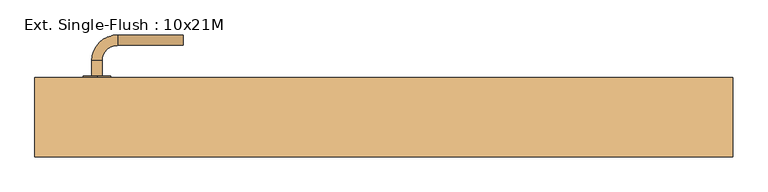
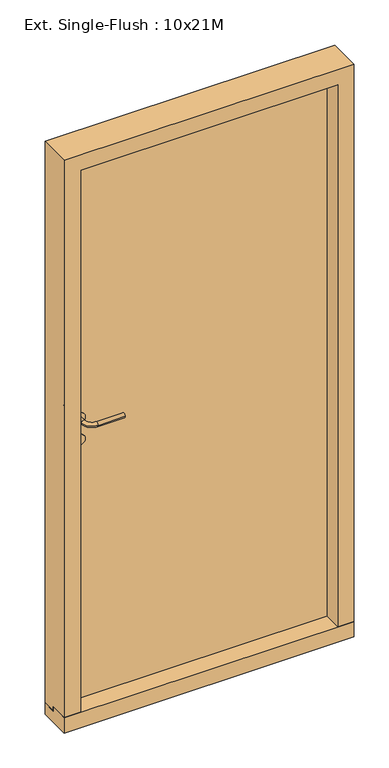
"""IFC4 building model written with IfcOpenShell, lengths in millimetres: door geometry, Ext. Single-Flush : 10x21M."""

import ifcopenshell
import ifcopenshell.guid

model = None  # the IFC model being written
_history = None  # IfcOwnerHistory: only IFC2X3 demands one
_inside = {}  # id of a spatial element -> (the spatial element, [elements in it])
_under = {}  # id of a project, library or spatial element -> (it, [spatial elements below it])
_declared = {}  # id of a project -> (the project, [libraries it declares])
_typed = {}  # id of a type object -> (the type object, [elements of that type])
_made_of = {}  # id of a material, layer set ... -> (it, [elements and type objects made of it])


def new_model(schema):
    """Start an empty IFC model of exactly this schema.

    Asked for "IFC4X3", IfcOpenShell would pick the latest addendum, in which some entities
    have other attributes; the version numbers below select the first issue.
    IFC2X3 requires an IfcOwnerHistory on every rooted entity: one is made here for all.
    """
    global model, _history
    if schema == "IFC4X3":
        model = ifcopenshell.file(schema_version=(4, 3, 0, 0))
    else:
        model = ifcopenshell.file(schema=schema)
    _inside.clear()
    _under.clear()
    _declared.clear()
    _typed.clear()
    _made_of.clear()
    _history = None
    if model.schema == "IFC2X3":
        org = make("IfcOrganization", Name="unknown")
        user = make(
            "IfcPersonAndOrganization",
            ThePerson=make("IfcPerson", FamilyName="unknown"),
            TheOrganization=org,
        )
        app = make(
            "IfcApplication",
            ApplicationDeveloper=org,
            Version="unknown",
            ApplicationFullName="unknown",
            ApplicationIdentifier="unknown",
        )
        _history = make(
            "IfcOwnerHistory",
            OwningUser=user,
            OwningApplication=app,
            ChangeAction="ADDED",
            CreationDate=0,
        )
    return model


def make(cls, **values):
    """One entity of the class cls with the attributes given. An attribute that is None is left unset."""
    return model.create_entity(
        cls, **{name: value for name, value in values.items() if value is not None}
    )


def rooted(cls, **values):
    """An entity with a GlobalId (a new one), such as an element, a storey or a relation."""
    return make(cls, GlobalId=ifcopenshell.guid.new(), OwnerHistory=_history, **values)


def si_unit(unit_type, name, prefix=None):
    """IfcSIUnit, for example si_unit("LENGTHUNIT", "METRE", prefix="MILLI")."""
    return make("IfcSIUnit", UnitType=unit_type, Prefix=prefix, Name=name)


def assignment(units):
    """IfcUnitAssignment: the units of a project."""
    return None if units is None else make("IfcUnitAssignment", Units=units)


def point(xyz):
    """IfcCartesianPoint."""
    return None if xyz is None else make("IfcCartesianPoint", Coordinates=xyz)


def direction(xyz):
    """IfcDirection."""
    return None if xyz is None else make("IfcDirection", DirectionRatios=xyz)


def frame(location, z_axis=None, x_axis=None):
    """IfcAxis2Placement3D, a coordinate frame: its origin and axes. An axis left out is left unset."""
    return make(
        "IfcAxis2Placement3D",
        Location=point(location),
        Axis=direction(z_axis),
        RefDirection=direction(x_axis),
    )


def frame_2d(location, x_axis=None):
    """IfcAxis2Placement2D, a coordinate frame in the plane: its origin and x axis."""
    return make(
        "IfcAxis2Placement2D", Location=point(location), RefDirection=direction(x_axis)
    )


def origin():
    """The frame at (0, 0, 0) with its axes left unset."""
    return frame((0.0, 0.0, 0.0))


def place(relative_to, where):
    """IfcLocalPlacement: puts the frame where relative to a parent placement (None: the world)."""
    return make(
        "IfcLocalPlacement", PlacementRelTo=relative_to, RelativePlacement=where
    )


def context(
    kind, dimensions, precision=None, world=None, true_north=None, identifier=None
):
    """IfcGeometricRepresentationContext, for example the 3D "Model" context."""
    return make(
        "IfcGeometricRepresentationContext",
        ContextIdentifier=identifier,
        ContextType=kind,
        CoordinateSpaceDimension=dimensions,
        Precision=precision,
        WorldCoordinateSystem=world,
        TrueNorth=true_north,
    )


def project(units=None, contexts=None):
    """IfcProject with its units and contexts."""
    return rooted(
        "IfcProject",
        Name="project",
        RepresentationContexts=contexts,
        UnitsInContext=assignment(units),
    )


def spatial(cls, under=None, at=None, **own):
    """A site, building, storey or space (cls), placed at a placement, below another one or the project."""
    s = rooted(cls, ObjectPlacement=at, **own)
    if under is not None:
        _under.setdefault(under.id(), (under, []))[1].append(s)
    return s


def polyline(points):
    """IfcPolyline through the points."""
    return make("IfcPolyline", Points=[point(p) for p in points])


def circle_curve(where, radius):
    """IfcCircle in the frame where."""
    return make("IfcCircle", Position=where, Radius=radius)


def ellipse_curve(where, semi_axis1, semi_axis2):
    """IfcEllipse in the frame where."""
    return make(
        "IfcEllipse", Position=where, SemiAxis1=semi_axis1, SemiAxis2=semi_axis2
    )


def trimmed(basis, trim1, trim2, sense, master):
    """IfcTrimmedCurve: the piece of a basis curve between two trims."""
    return make(
        "IfcTrimmedCurve",
        BasisCurve=basis,
        Trim1=trim1,
        Trim2=trim2,
        SenseAgreement=sense,
        MasterRepresentation=master,
    )


def segment(curve, same_sense, transition):
    """IfcCompositeCurveSegment."""
    return make(
        "IfcCompositeCurveSegment",
        Transition=transition,
        SameSense=same_sense,
        ParentCurve=curve,
    )


def composite_curve(segments, self_intersect=None):
    """IfcCompositeCurve: segments joined end to end."""
    return make("IfcCompositeCurve", Segments=segments, SelfIntersect=self_intersect)


def outline(outer, holes=None, kind="AREA"):
    """IfcArbitraryClosedProfileDef: a profile drawn as a closed curve; with holes, ...WithVoids."""
    if holes is None:
        return make("IfcArbitraryClosedProfileDef", ProfileType=kind, OuterCurve=outer)
    return make(
        "IfcArbitraryProfileDefWithVoids",
        ProfileType=kind,
        OuterCurve=outer,
        InnerCurves=holes,
    )


def extrude(swept, where, along, depth):
    """IfcExtrudedAreaSolid: the profile swept, set in the frame where, extruded along a direction by depth."""
    return make(
        "IfcExtrudedAreaSolid",
        SweptArea=swept,
        Position=where,
        ExtrudedDirection=direction(along),
        Depth=depth,
    )


def faces_of(points, faces, orient=None, outer=None):
    """IfcFace entities. A face is a list of loops; a loop is a list of indices into points, from 0.

    orient and outer hold one flag for each loop. By default every Orientation is true, the
    first loop of a face is its IfcFaceOuterBound and the others are IfcFaceBound.
    """
    made = []
    for i, loops in enumerate(faces):
        bounds = []
        for j, loop in enumerate(loops):
            is_outer = j == 0 if outer is None else outer[i][j]
            bounds.append(
                make(
                    "IfcFaceOuterBound" if is_outer else "IfcFaceBound",
                    Bound=make("IfcPolyLoop", Polygon=[points[k] for k in loop]),
                    Orientation=True if orient is None else orient[i][j],
                )
            )
        made.append(make("IfcFace", Bounds=bounds))
    return made


def faceted_brep(points, faces, orient=None, outer=None, voids=None):
    """IfcFacetedBrep: a solid bounded by flat faces; with voids (closed shells), ...WithVoids."""
    shared = [point(p) for p in points]
    hull = make("IfcClosedShell", CfsFaces=faces_of(shared, faces, orient, outer))
    if voids is None:
        return make("IfcFacetedBrep", Outer=hull)
    return make(
        "IfcFacetedBrepWithVoids",
        Outer=hull,
        Voids=[
            make(cls, CfsFaces=faces_of(shared, fs, o, b)) for cls, fs, o, b in voids
        ],
    )


def shape(context_of_items, identifier, shape_type, items):
    """IfcShapeRepresentation: the items that make up one representation, for example the "Body"."""
    return make(
        "IfcShapeRepresentation",
        ContextOfItems=context_of_items,
        RepresentationIdentifier=identifier,
        RepresentationType=shape_type,
        Items=items,
    )


def source(mapping_origin, context_of_items, identifier, shape_type, items):
    """IfcRepresentationMap: a shape defined once, which mapped items show again and again."""
    return make(
        "IfcRepresentationMap",
        MappingOrigin=mapping_origin,
        MappedRepresentation=shape(context_of_items, identifier, shape_type, items),
    )


def transform(
    local_origin,
    x_axis=None,
    y_axis=None,
    z_axis=None,
    scale=None,
    scale2=None,
    scale3=None,
    uniform=True,
):
    """IfcCartesianTransformationOperator3D, or its non-uniform kind. x_axis, y_axis, z_axis: its Axis1, 2, 3."""
    if uniform:
        return make(
            "IfcCartesianTransformationOperator3D",
            Axis1=direction(x_axis),
            Axis2=direction(y_axis),
            LocalOrigin=point(local_origin),
            Scale=scale,
            Axis3=direction(z_axis),
        )
    return make(
        "IfcCartesianTransformationOperator3DnonUniform",
        Axis1=direction(x_axis),
        Axis2=direction(y_axis),
        LocalOrigin=point(local_origin),
        Scale=scale,
        Axis3=direction(z_axis),
        Scale2=scale2,
        Scale3=scale3,
    )


def mapped(mapping_source, mapping_target):
    """IfcMappedItem: shows the shape of a source again, moved by a transform."""
    return make(
        "IfcMappedItem", MappingSource=mapping_source, MappingTarget=mapping_target
    )


def made_of(thing, what):
    """Note that an element or type object is made of a material, layer set ...; save() writes the relation."""
    if what is not None:
        _made_of.setdefault(what.id(), (what, []))[1].append(thing)
    return thing


def element(
    cls,
    number,
    at=None,
    inside=None,
    cuts=None,
    type_object=None,
    material=None,
    context=None,
    identifier="Body",
    shape_type=None,
    held_by="IfcProductDefinitionShape",
    body=None,
    shapes=None,
    **own,
):
    """One element of the class cls, such as IfcWall. Its Tag is "e" and its number.

    at: its placement. inside: the storey or other place that contains it. cuts: it is an
    opening in that element (IfcRelVoidsElement). A single representation is given by context,
    identifier, shape_type and body (its items); several are given by shapes. held_by: the class
    of the entity that holds the representations. save() writes the other relations.
    """
    e = rooted(cls, Tag="e%d" % number, ObjectPlacement=at, **own)
    if body is not None:
        shapes = [shape(context, identifier, shape_type, body)]
    if shapes is not None:
        e.Representation = make(held_by, Representations=shapes)
    if inside is not None:
        _inside.setdefault(inside.id(), (inside, []))[1].append(e)
    if cuts is not None:
        rooted(
            "IfcRelVoidsElement", RelatingBuildingElement=cuts, RelatedOpeningElement=e
        )
    if type_object is not None:
        _typed.setdefault(type_object.id(), (type_object, []))[1].append(e)
    return made_of(e, material)


def aggregate(whole, parts):
    """IfcRelAggregates: a whole, such as a stair, and the parts it consists of."""
    return rooted("IfcRelAggregates", RelatingObject=whole, RelatedObjects=parts)


def save(model, path):
    """Write the relations noted so far, then the file.

    IfcRelAggregates (storeys below a building ...), IfcRelContainedInSpatialStructure (elements
    in a storey), IfcRelDefinesByType, IfcRelAssociatesMaterial and IfcRelDeclares: one each for
    every whole, place, type object, material and project.
    """
    for whole, parts in _under.values():
        aggregate(whole, parts)
    for where, things in _inside.values():
        rooted(
            "IfcRelContainedInSpatialStructure",
            RelatedElements=things,
            RelatingStructure=where,
        )
    for kind, things in _typed.values():
        rooted("IfcRelDefinesByType", RelatedObjects=things, RelatingType=kind)
    for what, things in _made_of.values():
        rooted("IfcRelAssociatesMaterial", RelatedObjects=things, RelatingMaterial=what)
    for by, libraries in _declared.values():
        rooted("IfcRelDeclares", RelatingContext=by, RelatedDefinitions=libraries)
    model.write(path)


def plane_surface(at):
    """IfcPlane: the flat surface through the origin of the frame at, square to its z axis."""
    return make("IfcPlane", Position=at)


def cylinder_surface(at, radius):
    """IfcCylindricalSurface: all points at the distance radius from the z axis of the frame at."""
    return make("IfcCylindricalSurface", Position=at, Radius=radius)


def revolved_surface(curve, axis_point, axis_direction):
    """IfcSurfaceOfRevolution: the curve turned about the line through axis_point along axis_direction."""
    return make(
        "IfcSurfaceOfRevolution",
        SweptCurve=make("IfcArbitraryOpenProfileDef", ProfileType="CURVE", Curve=curve),
        AxisPosition=make("IfcAxis1Placement", Location=point(axis_point), Axis=direction(axis_direction)),
    )


def advanced_brep(points, edges, surfaces, faces):
    """IfcAdvancedBrep: a solid bounded by faces that lie on surfaces and meet in shared edges.

    An edge is (start, end): straight between two places in points (the first is 0);
    or (start, end, curve); or (start, end, curve, False) where it runs against its curve.
    A face is (place in surfaces, loops), or (place, loops, False) where it looks against
    its surface's normal. A loop lists edges by number (the first is 1), with a minus sign
    where the edge is run from its end to its start. The first loop is the outer one.
    """
    corners = [point(p) for p in points]
    vertices = [make("IfcVertexPoint", VertexGeometry=c) for c in corners]
    made = []
    for start, end, *more in edges:
        made.append(
            make(
                "IfcEdgeCurve",
                EdgeStart=vertices[start],
                EdgeEnd=vertices[end],
                EdgeGeometry=more[0] if more else make("IfcPolyline", Points=[corners[start], corners[end]]),
                SameSense=more[1] if len(more) > 1 else True,
            )
        )
    hull = []
    for where, loops, *sense in faces:
        bounds = []
        for j, loop in enumerate(loops):
            ring = [make("IfcOrientedEdge", EdgeElement=made[abs(k) - 1], Orientation=k > 0) for k in loop]
            bounds.append(
                make(
                    "IfcFaceOuterBound" if j == 0 else "IfcFaceBound",
                    Bound=make("IfcEdgeLoop", EdgeList=ring),
                    Orientation=True,
                )
            )
        hull.append(make("IfcAdvancedFace", Bounds=bounds, FaceSurface=surfaces[where], SameSense=sense[0] if sense else True))
    return make("IfcAdvancedBrep", Outer=make("IfcClosedShell", CfsFaces=hull))


def ext_single_flush_10x21m_d0052ec9(model_context):
    return source(origin(), model_context, "Body", "SolidModel", [
        extrude(outline(composite_curve([segment(trimmed(circle_curve(frame_2d((1090.0, -416.0)), 20.0), [point((1070.0, -416.0))], [point((1110.0, -416.0))], False, "CARTESIAN"), True, "CONTINUOUS"), segment(trimmed(circle_curve(frame_2d((1090.0, -416.0)), 20.0), [point((1110.0, -416.0))], [point((1070.0, -416.0))], False, "CARTESIAN"), True, "CONTINUOUS")], self_intersect=False)), frame((0.0, 184.0, 0.0), z_axis=(0.0, 1.0, 0.0), x_axis=(0.0, 0.0, 1.0)), (0.0, 0.0, 1.0), 2.0),
        advanced_brep(
        [(-423.5, 186.0, 1090.0), (-408.5, 186.0, 1090.0), (-423.5, 208.5, 1090.0), (-408.5, 208.5, 1090.0), (-386.0, 231.0, 1090.0), (-386.0, 246.0, 1090.0), (-291.0, 246.0, 1090.0), (-291.0, 231.0, 1090.0)],
        [
            (0, 1, circle_curve(frame((-416.0, 186.0, 1090.0), z_axis=(0.0, -1.0, 0.0), x_axis=(1.0, 0.0, 0.0)), 7.5)),
            (1, 0, circle_curve(frame((-416.0, 186.0, 1090.0), z_axis=(0.0, -1.0, 0.0), x_axis=(1.0, 0.0, 0.0)), 7.5)),
            (0, 2),
            (2, 3, circle_curve(frame((-416.0, 208.5, 1090.0), z_axis=(0.0, -1.0, 0.0), x_axis=(1.0, 0.0, 0.0)), 7.5)),
            (3, 1),
            (3, 2, circle_curve(frame((-416.0, 208.5, 1090.0), z_axis=(0.0, -1.0, 0.0), x_axis=(1.0, 0.0, 0.0)), 7.5)),
            (4, 3, circle_curve(frame((-386.0, 208.5, 1090.0), z_axis=(0.0, 0.0, 1.0), x_axis=(-1.0, 0.0, 0.0)), 22.5)),
            (2, 5, circle_curve(frame((-386.0, 208.5, 1090.0), z_axis=(0.0, 0.0, -1.0), x_axis=(-1.0, 0.0, 0.0)), 37.5)),
            (5, 4, circle_curve(frame((-386.0, 238.5, 1090.0), z_axis=(-1.0, 0.0, 0.0), x_axis=(0.0, -1.0, 0.0)), 7.5)),
            (4, 5, circle_curve(frame((-386.0, 238.5, 1090.0), z_axis=(-1.0, 0.0, 0.0), x_axis=(0.0, -1.0, 0.0)), 7.5)),
            (5, 6),
            (6, 7, circle_curve(frame((-291.0, 238.5, 1090.0), z_axis=(-1.0, 0.0, 0.0), x_axis=(0.0, -1.0, 0.0)), 7.5)),
            (7, 4),
            (7, 6, circle_curve(frame((-291.0, 238.5, 1090.0), z_axis=(-1.0, 0.0, 0.0), x_axis=(0.0, -1.0, 0.0)), 7.5)),
        ],
        [
            plane_surface(frame((-416.0, 186.0, 1090.0), z_axis=(0.0, -1.0, 0.0), x_axis=(0.0, 0.0, -1.0))),
            cylinder_surface(frame((-416.0, 186.0, 1090.0), z_axis=(0.0, -1.0, 0.0), x_axis=(1.0, 0.0, 0.0)), 7.5),
            revolved_surface(trimmed(ellipse_curve(frame((-416.0, 208.5, 1090.0), z_axis=(0.0, -1.0, 0.0), x_axis=(1.0, 0.0, 0.0)), 7.5, 7.5), [point((-423.5, 208.5, 1090.0))], [point((-408.5, 208.5, 1090.0))], True, "CARTESIAN"), (-386.0, 208.5, 1090.0), (0.0, 0.0, -1.0)),
            revolved_surface(trimmed(ellipse_curve(frame((-416.0, 208.5, 1090.0), z_axis=(0.0, -1.0, 0.0), x_axis=(1.0, 0.0, 0.0)), 7.5, 7.5), [point((-408.5, 208.5, 1090.0))], [point((-423.5, 208.5, 1090.0))], True, "CARTESIAN"), (-386.0, 208.5, 1090.0), (0.0, 0.0, -1.0)),
            cylinder_surface(frame((-386.0, 238.5, 1090.0), z_axis=(-1.0, 0.0, 0.0), x_axis=(0.0, -1.0, 0.0)), 7.5),
            plane_surface(frame((-291.0, 238.5, 1090.0), z_axis=(1.0, 0.0, 0.0), x_axis=(0.0, 0.0, -1.0))),
        ],
        [
            (0, [[1, 2]]),
            (1, [[-1, 3, 4, 5]]),
            (1, [[-2, -5, 6, -3]]),
            (2, [[7, -4, 8, 9]]),
            (3, [[-8, -6, -7, 10]]),
            (4, [[-9, 11, 12, 13]]),
            (4, [[-10, -13, 14, -11]]),
            (5, [[-14, -12]]),
        ],
    ),
        extrude(outline(composite_curve([segment(trimmed(circle_curve(frame_2d((1010.0, -416.0)), 20.0), [point((990.0, -416.0))], [point((1030.0, -416.0))], False, "CARTESIAN"), True, "CONTINUOUS"), segment(trimmed(circle_curve(frame_2d((1010.0, -416.0)), 20.0), [point((1030.0, -416.0))], [point((990.0, -416.0))], False, "CARTESIAN"), True, "CONTINUOUS")], self_intersect=False), holes=[composite_curve([segment(trimmed(circle_curve(frame_2d((1015.0, -416.0)), 3.0), [point((1012.4019238, -417.5))], [point((1012.4019238, -414.5))], True, "CARTESIAN"), True, "CONTINUOUS"), segment(polyline([(1012.4019238, -414.5), (1000.0, -414.5), (1000.0, -417.5), (1012.4019238, -417.5)]), True, "CONTINUOUS")], self_intersect=False)]), frame((0.0, 184.0, 0.0), z_axis=(0.0, 1.0, 0.0), x_axis=(0.0, 0.0, 1.0)), (0.0, 0.0, 1.0), 2.0),
        extrude(outline(composite_curve([segment(trimmed(circle_curve(frame_2d((1090.0, -416.0)), 20.0), [point((1070.0, -416.0))], [point((1110.0, -416.0))], False, "CARTESIAN"), True, "CONTINUOUS"), segment(trimmed(circle_curve(frame_2d((1090.0, -416.0)), 20.0), [point((1110.0, -416.0))], [point((1070.0, -416.0))], False, "CARTESIAN"), True, "CONTINUOUS")], self_intersect=False)), frame((0.0, 132.0, 0.0), z_axis=(0.0, 1.0, 0.0), x_axis=(0.0, 0.0, 1.0)), (0.0, 0.0, 1.0), 2.0),
        advanced_brep(
        [(-423.5, 132.0, 1090.0), (-408.5, 132.0, 1090.0), (-408.5, 109.5, 1090.0), (-423.5, 109.5, 1090.0), (-386.0, 87.0, 1090.0), (-386.0, 72.0, 1090.0), (-291.0, 87.0, 1090.0), (-291.0, 72.0, 1090.0)],
        [
            (0, 1, circle_curve(frame((-416.0, 132.0, 1090.0), z_axis=(0.0, 1.0, 0.0), x_axis=(1.0, 0.0, 0.0)), 7.5)),
            (1, 0, circle_curve(frame((-416.0, 132.0, 1090.0), z_axis=(0.0, 1.0, 0.0), x_axis=(1.0, 0.0, 0.0)), 7.5)),
            (1, 2),
            (2, 3, circle_curve(frame((-416.0, 109.5, 1090.0), z_axis=(0.0, 1.0, 0.0), x_axis=(1.0, 0.0, 0.0)), 7.5)),
            (3, 0),
            (3, 2, circle_curve(frame((-416.0, 109.5, 1090.0), z_axis=(0.0, 1.0, 0.0), x_axis=(1.0, 0.0, 0.0)), 7.5)),
            (4, 5, circle_curve(frame((-386.0, 79.5, 1090.0), z_axis=(-1.0, 0.0, 0.0), x_axis=(0.0, 1.0, 0.0)), 7.5)),
            (5, 3, circle_curve(frame((-386.0, 109.5, 1090.0), z_axis=(0.0, 0.0, -1.0), x_axis=(-1.0, 0.0, 0.0)), 37.5)),
            (2, 4, circle_curve(frame((-386.0, 109.5, 1090.0), z_axis=(0.0, 0.0, 1.0), x_axis=(-1.0, 0.0, 0.0)), 22.5)),
            (5, 4, circle_curve(frame((-386.0, 79.5, 1090.0), z_axis=(-1.0, 0.0, 0.0), x_axis=(0.0, 1.0, 0.0)), 7.5)),
            (4, 6),
            (6, 7, circle_curve(frame((-291.0, 79.5, 1090.0), z_axis=(-1.0, 0.0, 0.0), x_axis=(0.0, 1.0, 0.0)), 7.5)),
            (7, 5),
            (7, 6, circle_curve(frame((-291.0, 79.5, 1090.0), z_axis=(-1.0, 0.0, 0.0), x_axis=(0.0, 1.0, 0.0)), 7.5)),
        ],
        [
            plane_surface(frame((-416.0, 132.0, 1090.0), z_axis=(0.0, 1.0, 0.0), x_axis=(0.0, 0.0, -1.0))),
            cylinder_surface(frame((-416.0, 132.0, 1090.0), z_axis=(0.0, 1.0, 0.0), x_axis=(1.0, 0.0, 0.0)), 7.5),
            revolved_surface(trimmed(ellipse_curve(frame((-416.0, 109.5, 1090.0), z_axis=(0.0, -1.0, 0.0), x_axis=(1.0, 0.0, 0.0)), 7.5, 7.5), [point((-423.5, 109.5, 1090.0))], [point((-408.5, 109.5, 1090.0))], True, "CARTESIAN"), (-386.0, 109.5, 1090.0), (0.0, 0.0, -1.0)),
            revolved_surface(trimmed(ellipse_curve(frame((-416.0, 109.5, 1090.0), z_axis=(0.0, -1.0, 0.0), x_axis=(1.0, 0.0, 0.0)), 7.5, 7.5), [point((-408.5, 109.5, 1090.0))], [point((-423.5, 109.5, 1090.0))], True, "CARTESIAN"), (-386.0, 109.5, 1090.0), (0.0, 0.0, -1.0)),
            cylinder_surface(frame((-386.0, 79.5, 1090.0), z_axis=(-1.0, 0.0, 0.0), x_axis=(0.0, 1.0, 0.0)), 7.5),
            plane_surface(frame((-291.0, 79.5, 1090.0), z_axis=(1.0, 0.0, 0.0), x_axis=(0.0, 0.0, -1.0))),
        ],
        [
            (0, [[1, 2]]),
            (1, [[3, 4, 5, -2]]),
            (1, [[-5, 6, -3, -1]]),
            (2, [[7, 8, -4, 9]]),
            (3, [[10, -9, -6, -8]]),
            (4, [[11, 12, 13, -7]]),
            (4, [[-13, 14, -11, -10]]),
            (5, [[-12, -14]]),
        ],
    ),
        extrude(outline(composite_curve([segment(trimmed(circle_curve(frame_2d((1010.0, -416.0)), 20.0), [point((990.0, -416.0))], [point((1030.0, -416.0))], False, "CARTESIAN"), True, "CONTINUOUS"), segment(trimmed(circle_curve(frame_2d((1010.0, -416.0)), 20.0), [point((1030.0, -416.0))], [point((990.0, -416.0))], False, "CARTESIAN"), True, "CONTINUOUS")], self_intersect=False), holes=[composite_curve([segment(trimmed(circle_curve(frame_2d((1015.0, -416.0)), 3.0), [point((1012.4019238, -417.5))], [point((1012.4019238, -414.5))], True, "CARTESIAN"), True, "CONTINUOUS"), segment(polyline([(1012.4019238, -414.5), (1000.0, -414.5), (1000.0, -417.5), (1012.4019238, -417.5)]), True, "CONTINUOUS")], self_intersect=False)]), frame((0.0, 132.0, 0.0), z_axis=(0.0, 1.0, 0.0), x_axis=(0.0, 0.0, 1.0)), (0.0, 0.0, 1.0), 2.0),
        extrude(outline(polyline([(184.0, 42.0), (184.0, 0.0), (69.0, 0.0), (69.0, 57.0), (134.0, 57.0), (134.0, 42.0), (184.0, 42.0)])), frame((-506.0, 0.0, 0.0), z_axis=(1.0, 0.0, 0.0), x_axis=(0.0, 1.0, 0.0)), (0.0, 0.0, 1.0), 1012.0),
        extrude(outline(polyline([(-464.0, 184.0), (464.0, 184.0), (464.0, 134.0), (-464.0, 134.0), (-464.0, 184.0)])), frame((0.0, 0.0, 42.0), z_axis=(0.0, 0.0, 1.0), x_axis=(1.0, 0.0, 0.0)), (0.0, 0.0, 1.0), 2028.0),
        faceted_brep([(464.0, 184.0, 2070.0), (-464.0, 184.0, 2070.0), (-464.0, 184.0, 42.0), (-506.0, 184.0, 42.0), (-506.0, 184.0, 2112.0), (506.0, 184.0, 2112.0), (506.0, 184.0, 42.0), (464.0, 184.0, 42.0), (-464.0, 134.0, 2070.0), (-464.0, 134.0, 57.0), (-464.0, 134.0, 42.0), (506.0, 134.0, 42.0), (464.0, 134.0, 42.0), (-506.0, 134.0, 42.0), (-506.0, 69.0, 2112.0), (-506.0, 134.0, 57.0), (-506.0, 69.0, 57.0), (506.0, 69.0, 2112.0), (506.0, 69.0, 57.0), (506.0, 134.0, 57.0), (464.0, 134.0, 2070.0), (464.0, 134.0, 57.0), (-449.0, 69.0, 57.0), (-449.0, 69.0, 2055.0), (449.0, 69.0, 2055.0), (449.0, 69.0, 57.0), (449.0, 134.0, 57.0), (-449.0, 134.0, 57.0), (-449.0, 134.0, 2055.0), (449.0, 134.0, 2055.0)], [[[0, 1, 2, 3, 4, 5, 6, 7]], [[1, 8, 9, 10, 2]], [[11, 12, 7, 6]], [[10, 13, 3, 2]], [[14, 4, 3, 13, 15, 16]], [[5, 17, 18, 19, 11, 6]], [[20, 0, 7, 12, 21]], [[17, 14, 16, 22, 23, 24, 25, 18]], [[21, 19, 18, 25, 26]], [[15, 9, 27, 22, 16]], [[19, 21, 12, 11]], [[9, 15, 13, 10]], [[28, 23, 22, 27]], [[24, 29, 26, 25]], [[29, 28, 27, 9, 8, 20, 21, 26]], [[5, 4, 14, 17]], [[24, 23, 28, 29]], [[1, 0, 20, 8]]]),
    ])


if __name__ == "__main__":
    model = new_model("IFC4")
    model_context = context("Model", 3, world=origin())
    ifc_project = project(units=[si_unit("LENGTHUNIT", "METRE", prefix="MILLI")], contexts=[model_context])
    site = spatial("IfcSite", under=ifc_project)
    building = spatial("IfcBuilding", under=site)
    placement = place(None, origin())
    ext_single_flush_10x21m_shape = ext_single_flush_10x21m_d0052ec9(model_context)
    element("IfcDoor", 1, ObjectType="Ext. Single-Flush : 10x21M", at=placement, inside=building, context=model_context, shape_type="MappedRepresentation", body=[
        mapped(ext_single_flush_10x21m_shape, transform((0.0, 0.0, 0.0), x_axis=(1.0, 0.0, 0.0), y_axis=(0.0, 1.0, 0.0), z_axis=(0.0, 0.0, 1.0))),
    ])
    save(model, "model.ifc")

# Revit data of these elements
# Type "Ext. Single-Flush : 10x21M"
#   Type Mark = "52"
#   Sound Rating = ""
#   Opening Side [instance default] = ""
#   Hinge Side [instance default] = ""
#   Creator Organization [instance default] = "© Danish Educational Content"
#   Creator Name [instance default] = "© Erik Falck Jørgensen"
#   Creator Build [instance default] = "2017.0801.0"
#   Analytic Construction = "<None>"
#   length#7 = -50 mm
#   length#6 = 1012 mm
#   length#5 = 120 mm
#   length#4 = 42 mm
#   length#3 = 57 mm
#   length#2a = 0 mm
#   length#2 = 0 mm
#   length#1 = 0 mm
#   Thickness = 50 mm
#   Seal Width = 12 mm
#   Rough Width = 1012 mm
#   Rough Height = 2112 mm
#   Rebate Depth = 50 mm
#   Rabbet Depth = 50 mm
#   Height = 2088 mm
#   Width = 988 mm
#   Handle From Side = 90 mm
#   Handle From Bottom = 1090 mm
#   Exterior Direction [instance default] = 0.00°
#   Case Width = 45 mm
#   Rabbet Width = 15 mm
#   Case Depth = 115 mm
#   Bottom Seal = 12 mm
#   Threshold = yes
#   Sealing = no
#   Hinging = yes
#   Wall Closure = 1
#   Function = 1
#   Panel = none
#   Handle Finish = none
#   Handle = element 507533
#   Embrasure Interior = none
#   Embrasure Exterior = none
#   Case/Transom = none
#   Assembly Code = ""
# Element 1 (IfcDoor, "Ext. Single-Flush : 10x21M")
#   Materials on its faces: "Stainless Steel, Polished", "Default Frame/Mullion (Interior/Exterior)", "Default Door Panel (Exterior/Interior)"
# Materials
#   "Stainless Steel, Polished": class "Metal", colour RGB 180 180 180, transparency 0, Description = "Rustfri stål, poleret", Cost = 0
#   "Default Frame/Mullion (Interior/Exterior)": class "Generic", colour RGB 205 205 205, transparency 0, Description = "Udefineret karm/ramme materiale", Cost = 0
#   "Default Door Panel (Exterior/Interior)": class "Generic", colour RGB 205 205 205, transparency 0, Description = "Udefineret dørplade materiale", Cost = 0
